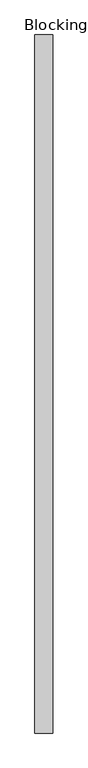
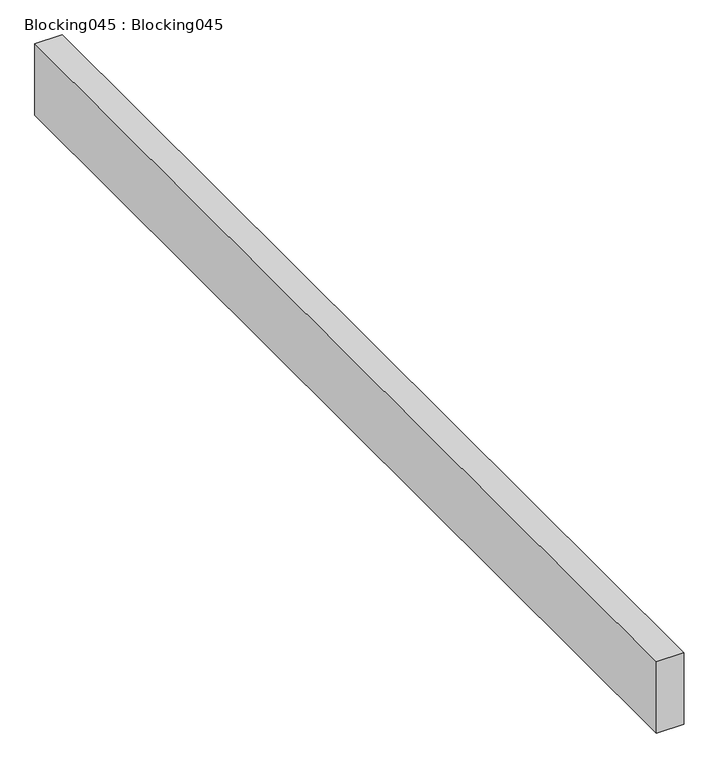
"""IFC4 building model written with IfcOpenShell, lengths in millimetres: proxy geometry, Blocking045 : Blocking045."""

from ifc_helpers import new_model, si_unit, frame, origin, place, context, project, spatial, polyline, outline, extrude, source, transform, mapped, element, save


def blocking045_blocking045_0cd26f1d(model_context):
    return source(origin(), model_context, "Body", "SweptSolid", [
        extrude(outline(polyline([(-4423.2538825, -1052.8908936), (-4474.0538825, -1052.8908936), (-4474.0538825, 947.1091064), (-4423.2538825, 947.1091064), (-4423.2538825, -1052.8908936)])), frame((0.0, 0.0, 39972.996), z_axis=(0.0, 0.0, 1.0), x_axis=(1.0, 0.0, 0.0)), (0.0, 0.0, 1.0), 139.7),
    ])


if __name__ == "__main__":
    model = new_model("IFC4")
    model_context = context("Model", 3, world=origin())
    ifc_project = project(units=[si_unit("LENGTHUNIT", "METRE", prefix="MILLI")], contexts=[model_context])
    site = spatial("IfcSite", under=ifc_project)
    building = spatial("IfcBuilding", under=site)
    placement = place(None, origin())
    blocking045_blocking045_shape = blocking045_blocking045_0cd26f1d(model_context)
    element("IfcBuildingElementProxy", 1, Name="Blocking045 : Blocking045", ObjectType="Blocking045 : Blocking045", at=placement, inside=building, context=model_context, shape_type="MappedRepresentation", body=[
        mapped(blocking045_blocking045_shape, transform((0.0, 0.0, 0.0), x_axis=(1.0, 0.0, 0.0), y_axis=(0.0, 1.0, 0.0), z_axis=(0.0, 0.0, 1.0))),
    ])
    save(model, "model.ifc")

# Revit data of these elements
# Type "Blocking045 : Blocking045"
#   NameOverride = "Blocking045"
# Element 1 (IfcBuildingElementProxy, "Blocking045 : Blocking045")
#   Materials on its faces: "WOOD BLOCKING AS REQUIRED"
# Materials
#   "WOOD BLOCKING AS REQUIRED": class "Unassigned", colour RGB 166 124 85, transparency 0, Cost = 0
